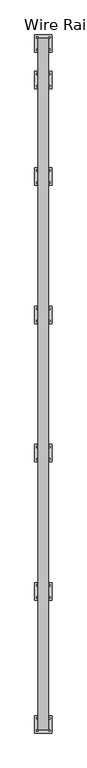
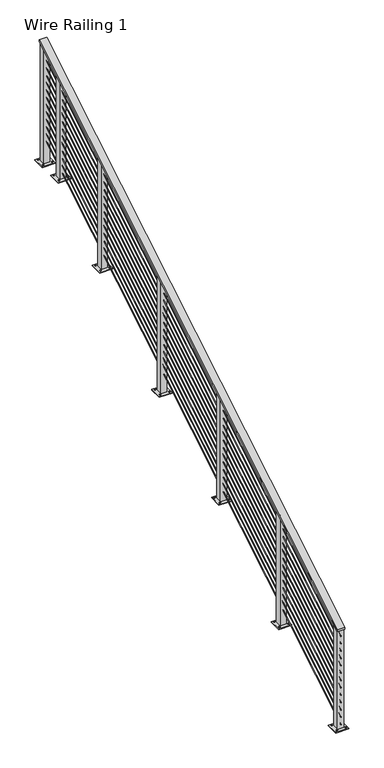
"""IFC4 building model written with IfcOpenShell, lengths in millimetres: railing geometry, Wire Railing 1."""

from ifc_helpers import new_model, si_unit, point, frame, frame_2d, origin, place, context, project, spatial, polyline, circle_curve, ellipse_curve, trimmed, segment, composite_curve, outline, extrude, faceted_brep, source, transform, mapped, element, save
from ifc_brep_helpers import plane_surface, cylinder_surface, advanced_brep


def wire_railing_1_93458223(model_context):
    return source(origin(), model_context, "Body", "SolidModel", [
        faceted_brep([(33186.6840778, 30205.3668167, 267463.590833), (33186.6840778, 30205.3668167, 267441.359167), (33262.8840778, 30205.3668167, 267441.359167), (33262.8840778, 30205.3668167, 267463.590833), (33186.6840778, 35259.9668167, 270504.4598169), (33262.8840778, 35259.9668167, 270504.4598169), (33262.8840778, 35259.9668167, 270482.228151), (33186.6840778, 35259.9668167, 270482.228151)], [[[0, 1, 2, 3]], [[4, 5, 6, 7]], [[1, 0, 4, 7]], [[2, 1, 7, 6]], [[3, 2, 6, 5]], [[0, 3, 5, 4]]]),
        advanced_brep(
        [(33227.1653278, 30205.3668167, 267383.0210418), (33222.4028278, 30205.3668167, 267383.0210418), (33227.1653278, 35259.9668167, 270423.8900257), (33222.4028278, 35259.9668167, 270423.8900257)],
        [
            (0, 1, ellipse_curve(frame((33224.7840778, 30205.3668167, 267383.0210418), z_axis=(0.0, -1.0, 0.0), x_axis=(0.0, 0.0, -1.0)), 2.7789582, 2.38125)),
            (1, 0, ellipse_curve(frame((33224.7840778, 30205.3668167, 267383.0210418), z_axis=(0.0, -1.0, 0.0), x_axis=(0.0, 0.0, -1.0)), 2.7789582, 2.38125)),
            (2, 3, ellipse_curve(frame((33224.7840778, 35259.9668167, 270423.8900257), z_axis=(0.0, 1.0, 0.0), x_axis=(0.0, 0.0, -1.0)), 2.7789582, 2.38125)),
            (3, 2, ellipse_curve(frame((33224.7840778, 35259.9668167, 270423.8900257), z_axis=(0.0, 1.0, 0.0), x_axis=(0.0, 0.0, -1.0)), 2.7789582, 2.38125)),
            (0, 2),
            (3, 1),
        ],
        [
            plane_surface(frame((33224.7840778, 30205.3668167, 267385.8), z_axis=(0.0, -1.0, 0.0), x_axis=(0.0, 0.0, 1.0))),
            plane_surface(frame((33224.7840778, 35259.9668167, 270426.668984), z_axis=(0.0, 1.0, 0.0), x_axis=(0.0, 0.0, 1.0))),
            cylinder_surface(frame((33224.7840778, 30206.5943658, 267383.7595406), z_axis=(0.0, -0.8568858520826472, -0.5155061944347475), x_axis=(-1.0, 0.0, 0.0)), 2.38125),
        ],
        [
            (0, [[1, 2]]),
            (1, [[3, 4]]),
            (2, [[-1, 5, -4, 6]]),
            (2, [[-2, -6, -3, -5]]),
        ],
    ),
        advanced_brep(
        [(33227.1653278, 30205.3668167, 267306.8210418), (33222.4028278, 30205.3668167, 267306.8210418), (33227.1653278, 35259.9668167, 270347.6900257), (33222.4028278, 35259.9668167, 270347.6900257)],
        [
            (0, 1, ellipse_curve(frame((33224.7840778, 30205.3668167, 267306.8210418), z_axis=(0.0, -1.0, 0.0), x_axis=(0.0, 0.0, -1.0)), 2.7789582, 2.38125)),
            (1, 0, ellipse_curve(frame((33224.7840778, 30205.3668167, 267306.8210418), z_axis=(0.0, -1.0, 0.0), x_axis=(0.0, 0.0, -1.0)), 2.7789582, 2.38125)),
            (2, 3, ellipse_curve(frame((33224.7840778, 35259.9668167, 270347.6900257), z_axis=(0.0, 1.0, 0.0), x_axis=(0.0, 0.0, -1.0)), 2.7789582, 2.38125)),
            (3, 2, ellipse_curve(frame((33224.7840778, 35259.9668167, 270347.6900257), z_axis=(0.0, 1.0, 0.0), x_axis=(0.0, 0.0, -1.0)), 2.7789582, 2.38125)),
            (0, 2),
            (3, 1),
        ],
        [
            plane_surface(frame((33224.7840778, 30205.3668167, 267309.6), z_axis=(0.0, -1.0, 0.0), x_axis=(0.0, 0.0, 1.0))),
            plane_surface(frame((33224.7840778, 35259.9668167, 270350.468984), z_axis=(0.0, 1.0, 0.0), x_axis=(0.0, 0.0, 1.0))),
            cylinder_surface(frame((33224.7840778, 30206.5943658, 267307.5595406), z_axis=(0.0, -0.8568858520826472, -0.5155061944347475), x_axis=(-1.0, 0.0, 0.0)), 2.38125),
        ],
        [
            (0, [[1, 2]]),
            (1, [[3, 4]]),
            (2, [[-1, 5, -4, 6]]),
            (2, [[-2, -6, -3, -5]]),
        ],
    ),
        advanced_brep(
        [(33227.1653278, 30205.3668167, 267230.6210418), (33222.4028278, 30205.3668167, 267230.6210418), (33227.1653278, 35259.9668167, 270271.4900257), (33222.4028278, 35259.9668167, 270271.4900257)],
        [
            (0, 1, ellipse_curve(frame((33224.7840778, 30205.3668167, 267230.6210418), z_axis=(0.0, -1.0, 0.0), x_axis=(0.0, 0.0, -1.0)), 2.7789582, 2.38125)),
            (1, 0, ellipse_curve(frame((33224.7840778, 30205.3668167, 267230.6210418), z_axis=(0.0, -1.0, 0.0), x_axis=(0.0, 0.0, -1.0)), 2.7789582, 2.38125)),
            (2, 3, ellipse_curve(frame((33224.7840778, 35259.9668167, 270271.4900257), z_axis=(0.0, 1.0, 0.0), x_axis=(0.0, 0.0, -1.0)), 2.7789582, 2.38125)),
            (3, 2, ellipse_curve(frame((33224.7840778, 35259.9668167, 270271.4900257), z_axis=(0.0, 1.0, 0.0), x_axis=(0.0, 0.0, -1.0)), 2.7789582, 2.38125)),
            (0, 2),
            (3, 1),
        ],
        [
            plane_surface(frame((33224.7840778, 30205.3668167, 267233.4), z_axis=(0.0, -1.0, 0.0), x_axis=(0.0, 0.0, 1.0))),
            plane_surface(frame((33224.7840778, 35259.9668167, 270274.268984), z_axis=(0.0, 1.0, 0.0), x_axis=(0.0, 0.0, 1.0))),
            cylinder_surface(frame((33224.7840778, 30206.5943658, 267231.3595406), z_axis=(0.0, -0.8568858520826472, -0.5155061944347475), x_axis=(-1.0, 0.0, 0.0)), 2.38125),
        ],
        [
            (0, [[1, 2]]),
            (1, [[3, 4]]),
            (2, [[-1, 5, -4, 6]]),
            (2, [[-2, -6, -3, -5]]),
        ],
    ),
        advanced_brep(
        [(33227.1653278, 30205.3668167, 267154.4210418), (33222.4028278, 30205.3668167, 267154.4210418), (33227.1653278, 35259.9668167, 270195.2900257), (33222.4028278, 35259.9668167, 270195.2900257)],
        [
            (0, 1, ellipse_curve(frame((33224.7840778, 30205.3668167, 267154.4210418), z_axis=(0.0, -1.0, 0.0), x_axis=(0.0, 0.0, -1.0)), 2.7789582, 2.38125)),
            (1, 0, ellipse_curve(frame((33224.7840778, 30205.3668167, 267154.4210418), z_axis=(0.0, -1.0, 0.0), x_axis=(0.0, 0.0, -1.0)), 2.7789582, 2.38125)),
            (2, 3, ellipse_curve(frame((33224.7840778, 35259.9668167, 270195.2900257), z_axis=(0.0, 1.0, 0.0), x_axis=(0.0, 0.0, -1.0)), 2.7789582, 2.38125)),
            (3, 2, ellipse_curve(frame((33224.7840778, 35259.9668167, 270195.2900257), z_axis=(0.0, 1.0, 0.0), x_axis=(0.0, 0.0, -1.0)), 2.7789582, 2.38125)),
            (0, 2),
            (3, 1),
        ],
        [
            plane_surface(frame((33224.7840778, 30205.3668167, 267157.2), z_axis=(0.0, -1.0, 0.0), x_axis=(0.0, 0.0, 1.0))),
            plane_surface(frame((33224.7840778, 35259.9668167, 270198.068984), z_axis=(0.0, 1.0, 0.0), x_axis=(0.0, 0.0, 1.0))),
            cylinder_surface(frame((33224.7840778, 30206.5943658, 267155.1595406), z_axis=(0.0, -0.8568858520826472, -0.5155061944347475), x_axis=(-1.0, 0.0, 0.0)), 2.38125),
        ],
        [
            (0, [[1, 2]]),
            (1, [[3, 4]]),
            (2, [[-1, 5, -4, 6]]),
            (2, [[-2, -6, -3, -5]]),
        ],
    ),
        advanced_brep(
        [(33227.1653278, 30205.3668167, 267078.2210418), (33222.4028278, 30205.3668167, 267078.2210418), (33227.1653278, 35259.9668167, 270119.0900257), (33222.4028278, 35259.9668167, 270119.0900257)],
        [
            (0, 1, ellipse_curve(frame((33224.7840778, 30205.3668167, 267078.2210418), z_axis=(0.0, -1.0, 0.0), x_axis=(0.0, 0.0, -1.0)), 2.7789582, 2.38125)),
            (1, 0, ellipse_curve(frame((33224.7840778, 30205.3668167, 267078.2210418), z_axis=(0.0, -1.0, 0.0), x_axis=(0.0, 0.0, -1.0)), 2.7789582, 2.38125)),
            (2, 3, ellipse_curve(frame((33224.7840778, 35259.9668167, 270119.0900257), z_axis=(0.0, 1.0, 0.0), x_axis=(0.0, 0.0, -1.0)), 2.7789582, 2.38125)),
            (3, 2, ellipse_curve(frame((33224.7840778, 35259.9668167, 270119.0900257), z_axis=(0.0, 1.0, 0.0), x_axis=(0.0, 0.0, -1.0)), 2.7789582, 2.38125)),
            (0, 2),
            (3, 1),
        ],
        [
            plane_surface(frame((33224.7840778, 30205.3668167, 267081.0), z_axis=(0.0, -1.0, 0.0), x_axis=(0.0, 0.0, 1.0))),
            plane_surface(frame((33224.7840778, 35259.9668167, 270121.868984), z_axis=(0.0, 1.0, 0.0), x_axis=(0.0, 0.0, 1.0))),
            cylinder_surface(frame((33224.7840778, 30206.5943658, 267078.9595406), z_axis=(0.0, -0.8568858520826472, -0.5155061944347475), x_axis=(-1.0, 0.0, 0.0)), 2.38125),
        ],
        [
            (0, [[1, 2]]),
            (1, [[3, 4]]),
            (2, [[-1, 5, -4, 6]]),
            (2, [[-2, -6, -3, -5]]),
        ],
    ),
        advanced_brep(
        [(33227.1653278, 30205.3668167, 267002.0210418), (33222.4028278, 30205.3668167, 267002.0210418), (33227.1653278, 35259.9668167, 270042.8900257), (33222.4028278, 35259.9668167, 270042.8900257)],
        [
            (0, 1, ellipse_curve(frame((33224.7840778, 30205.3668167, 267002.0210418), z_axis=(0.0, -1.0, 0.0), x_axis=(0.0, 0.0, -1.0)), 2.7789582, 2.38125)),
            (1, 0, ellipse_curve(frame((33224.7840778, 30205.3668167, 267002.0210418), z_axis=(0.0, -1.0, 0.0), x_axis=(0.0, 0.0, -1.0)), 2.7789582, 2.38125)),
            (2, 3, ellipse_curve(frame((33224.7840778, 35259.9668167, 270042.8900257), z_axis=(0.0, 1.0, 0.0), x_axis=(0.0, 0.0, -1.0)), 2.7789582, 2.38125)),
            (3, 2, ellipse_curve(frame((33224.7840778, 35259.9668167, 270042.8900257), z_axis=(0.0, 1.0, 0.0), x_axis=(0.0, 0.0, -1.0)), 2.7789582, 2.38125)),
            (0, 2),
            (3, 1),
        ],
        [
            plane_surface(frame((33224.7840778, 30205.3668167, 267004.8), z_axis=(0.0, -1.0, 0.0), x_axis=(0.0, 0.0, 1.0))),
            plane_surface(frame((33224.7840778, 35259.9668167, 270045.668984), z_axis=(0.0, 1.0, 0.0), x_axis=(0.0, 0.0, 1.0))),
            cylinder_surface(frame((33224.7840778, 30206.5943658, 267002.7595406), z_axis=(0.0, -0.8568858520826472, -0.5155061944347475), x_axis=(-1.0, 0.0, 0.0)), 2.38125),
        ],
        [
            (0, [[1, 2]]),
            (1, [[3, 4]]),
            (2, [[-1, 5, -4, 6]]),
            (2, [[-2, -6, -3, -5]]),
        ],
    ),
        advanced_brep(
        [(33227.1653278, 30205.3668167, 266925.8210418), (33222.4028278, 30205.3668167, 266925.8210418), (33227.1653278, 35259.9668167, 269966.6900257), (33222.4028278, 35259.9668167, 269966.6900257)],
        [
            (0, 1, ellipse_curve(frame((33224.7840778, 30205.3668167, 266925.8210418), z_axis=(0.0, -1.0, 0.0), x_axis=(0.0, 0.0, -1.0)), 2.7789582, 2.38125)),
            (1, 0, ellipse_curve(frame((33224.7840778, 30205.3668167, 266925.8210418), z_axis=(0.0, -1.0, 0.0), x_axis=(0.0, 0.0, -1.0)), 2.7789582, 2.38125)),
            (2, 3, ellipse_curve(frame((33224.7840778, 35259.9668167, 269966.6900257), z_axis=(0.0, 1.0, 0.0), x_axis=(0.0, 0.0, -1.0)), 2.7789582, 2.38125)),
            (3, 2, ellipse_curve(frame((33224.7840778, 35259.9668167, 269966.6900257), z_axis=(0.0, 1.0, 0.0), x_axis=(0.0, 0.0, -1.0)), 2.7789582, 2.38125)),
            (0, 2),
            (3, 1),
        ],
        [
            plane_surface(frame((33224.7840778, 30205.3668167, 266928.6), z_axis=(0.0, -1.0, 0.0), x_axis=(0.0, 0.0, 1.0))),
            plane_surface(frame((33224.7840778, 35259.9668167, 269969.468984), z_axis=(0.0, 1.0, 0.0), x_axis=(0.0, 0.0, 1.0))),
            cylinder_surface(frame((33224.7840778, 30206.5943658, 266926.5595406), z_axis=(0.0, -0.8568858520826472, -0.5155061944347475), x_axis=(-1.0, 0.0, 0.0)), 2.38125),
        ],
        [
            (0, [[1, 2]]),
            (1, [[3, 4]]),
            (2, [[-1, 5, -4, 6]]),
            (2, [[-2, -6, -3, -5]]),
        ],
    ),
        advanced_brep(
        [(33227.1653278, 30205.3668167, 266849.6210418), (33222.4028278, 30205.3668167, 266849.6210418), (33227.1653278, 35259.9668167, 269890.4900257), (33222.4028278, 35259.9668167, 269890.4900257)],
        [
            (0, 1, ellipse_curve(frame((33224.7840778, 30205.3668167, 266849.6210418), z_axis=(0.0, -1.0, 0.0), x_axis=(0.0, 0.0, -1.0)), 2.7789582, 2.38125)),
            (1, 0, ellipse_curve(frame((33224.7840778, 30205.3668167, 266849.6210418), z_axis=(0.0, -1.0, 0.0), x_axis=(0.0, 0.0, -1.0)), 2.7789582, 2.38125)),
            (2, 3, ellipse_curve(frame((33224.7840778, 35259.9668167, 269890.4900257), z_axis=(0.0, 1.0, 0.0), x_axis=(0.0, 0.0, -1.0)), 2.7789582, 2.38125)),
            (3, 2, ellipse_curve(frame((33224.7840778, 35259.9668167, 269890.4900257), z_axis=(0.0, 1.0, 0.0), x_axis=(0.0, 0.0, -1.0)), 2.7789582, 2.38125)),
            (0, 2),
            (3, 1),
        ],
        [
            plane_surface(frame((33224.7840778, 30205.3668167, 266852.4), z_axis=(0.0, -1.0, 0.0), x_axis=(0.0, 0.0, 1.0))),
            plane_surface(frame((33224.7840778, 35259.9668167, 269893.268984), z_axis=(0.0, 1.0, 0.0), x_axis=(0.0, 0.0, 1.0))),
            cylinder_surface(frame((33224.7840778, 30206.5943658, 266850.3595406), z_axis=(0.0, -0.8568858520826472, -0.5155061944347475), x_axis=(-1.0, 0.0, 0.0)), 2.38125),
        ],
        [
            (0, [[1, 2]]),
            (1, [[3, 4]]),
            (2, [[-1, 5, -4, 6]]),
            (2, [[-2, -6, -3, -5]]),
        ],
    ),
        advanced_brep(
        [(33227.1653278, 30205.3668167, 266773.4210418), (33222.4028278, 30205.3668167, 266773.4210418), (33227.1653278, 35259.9668167, 269814.2900257), (33222.4028278, 35259.9668167, 269814.2900257)],
        [
            (0, 1, ellipse_curve(frame((33224.7840778, 30205.3668167, 266773.4210418), z_axis=(0.0, -1.0, 0.0), x_axis=(0.0, 0.0, -1.0)), 2.7789582, 2.38125)),
            (1, 0, ellipse_curve(frame((33224.7840778, 30205.3668167, 266773.4210418), z_axis=(0.0, -1.0, 0.0), x_axis=(0.0, 0.0, -1.0)), 2.7789582, 2.38125)),
            (2, 3, ellipse_curve(frame((33224.7840778, 35259.9668167, 269814.2900257), z_axis=(0.0, 1.0, 0.0), x_axis=(0.0, 0.0, -1.0)), 2.7789582, 2.38125)),
            (3, 2, ellipse_curve(frame((33224.7840778, 35259.9668167, 269814.2900257), z_axis=(0.0, 1.0, 0.0), x_axis=(0.0, 0.0, -1.0)), 2.7789582, 2.38125)),
            (0, 2),
            (3, 1),
        ],
        [
            plane_surface(frame((33224.7840778, 30205.3668167, 266776.2), z_axis=(0.0, -1.0, 0.0), x_axis=(0.0, 0.0, 1.0))),
            plane_surface(frame((33224.7840778, 35259.9668167, 269817.068984), z_axis=(0.0, 1.0, 0.0), x_axis=(0.0, 0.0, 1.0))),
            cylinder_surface(frame((33224.7840778, 30206.5943658, 266774.1595406), z_axis=(0.0, -0.8568858520826472, -0.5155061944347475), x_axis=(-1.0, 0.0, 0.0)), 2.38125),
        ],
        [
            (0, [[1, 2]]),
            (1, [[3, 4]]),
            (2, [[-1, 5, -4, 6]]),
            (2, [[-2, -6, -3, -5]]),
        ],
    ),
        advanced_brep(
        [(33227.1653278, 30205.3668167, 266697.2210418), (33222.4028278, 30205.3668167, 266697.2210418), (33227.1653278, 35259.9668167, 269738.0900257), (33222.4028278, 35259.9668167, 269738.0900257)],
        [
            (0, 1, ellipse_curve(frame((33224.7840778, 30205.3668167, 266697.2210418), z_axis=(0.0, -1.0, 0.0), x_axis=(0.0, 0.0, -1.0)), 2.7789582, 2.38125)),
            (1, 0, ellipse_curve(frame((33224.7840778, 30205.3668167, 266697.2210418), z_axis=(0.0, -1.0, 0.0), x_axis=(0.0, 0.0, -1.0)), 2.7789582, 2.38125)),
            (2, 3, ellipse_curve(frame((33224.7840778, 35259.9668167, 269738.0900257), z_axis=(0.0, 1.0, 0.0), x_axis=(0.0, 0.0, -1.0)), 2.7789582, 2.38125)),
            (3, 2, ellipse_curve(frame((33224.7840778, 35259.9668167, 269738.0900257), z_axis=(0.0, 1.0, 0.0), x_axis=(0.0, 0.0, -1.0)), 2.7789582, 2.38125)),
            (0, 2),
            (3, 1),
        ],
        [
            plane_surface(frame((33224.7840778, 30205.3668167, 266700.0), z_axis=(0.0, -1.0, 0.0), x_axis=(0.0, 0.0, 1.0))),
            plane_surface(frame((33224.7840778, 35259.9668167, 269740.868984), z_axis=(0.0, 1.0, 0.0), x_axis=(0.0, 0.0, 1.0))),
            cylinder_surface(frame((33224.7840778, 30206.5943658, 266697.9595406), z_axis=(0.0, -0.8568858520826472, -0.5155061944347475), x_axis=(-1.0, 0.0, 0.0)), 2.38125),
        ],
        [
            (0, [[1, 2]]),
            (1, [[3, 4]]),
            (2, [[-1, 5, -4, 6]]),
            (2, [[-2, -6, -3, -5]]),
        ],
    ),
        advanced_brep(
        [(33227.1653278, 30205.3668167, 266621.0210418), (33222.4028278, 30205.3668167, 266621.0210418), (33227.1653278, 35259.9668167, 269661.8900257), (33222.4028278, 35259.9668167, 269661.8900257)],
        [
            (0, 1, ellipse_curve(frame((33224.7840778, 30205.3668167, 266621.0210418), z_axis=(0.0, -1.0, 0.0), x_axis=(0.0, 0.0, -1.0)), 2.7789582, 2.38125)),
            (1, 0, ellipse_curve(frame((33224.7840778, 30205.3668167, 266621.0210418), z_axis=(0.0, -1.0, 0.0), x_axis=(0.0, 0.0, -1.0)), 2.7789582, 2.38125)),
            (2, 3, ellipse_curve(frame((33224.7840778, 35259.9668167, 269661.8900257), z_axis=(0.0, 1.0, 0.0), x_axis=(0.0, 0.0, -1.0)), 2.7789582, 2.38125)),
            (3, 2, ellipse_curve(frame((33224.7840778, 35259.9668167, 269661.8900257), z_axis=(0.0, 1.0, 0.0), x_axis=(0.0, 0.0, -1.0)), 2.7789582, 2.38125)),
            (0, 2),
            (3, 1),
        ],
        [
            plane_surface(frame((33224.7840778, 30205.3668167, 266623.8), z_axis=(0.0, -1.0, 0.0), x_axis=(0.0, 0.0, 1.0))),
            plane_surface(frame((33224.7840778, 35259.9668167, 269664.668984), z_axis=(0.0, 1.0, 0.0), x_axis=(0.0, 0.0, 1.0))),
            cylinder_surface(frame((33224.7840778, 30206.5943658, 266621.7595406), z_axis=(0.0, -0.8568858520826472, -0.5155061944347475), x_axis=(-1.0, 0.0, 0.0)), 2.38125),
        ],
        [
            (0, [[1, 2]]),
            (1, [[3, 4]]),
            (2, [[-1, 5, -4, 6]]),
            (2, [[-2, -6, -3, -5]]),
        ],
    ),
        advanced_brep(
        [(33227.1653278, 30205.3668167, 266544.8210418), (33222.4028278, 30205.3668167, 266544.8210418), (33227.1653278, 35259.9668167, 269585.6900257), (33222.4028278, 35259.9668167, 269585.6900257)],
        [
            (0, 1, ellipse_curve(frame((33224.7840778, 30205.3668167, 266544.8210418), z_axis=(0.0, -1.0, 0.0), x_axis=(0.0, 0.0, -1.0)), 2.7789582, 2.38125)),
            (1, 0, ellipse_curve(frame((33224.7840778, 30205.3668167, 266544.8210418), z_axis=(0.0, -1.0, 0.0), x_axis=(0.0, 0.0, -1.0)), 2.7789582, 2.38125)),
            (2, 3, ellipse_curve(frame((33224.7840778, 35259.9668167, 269585.6900257), z_axis=(0.0, 1.0, 0.0), x_axis=(0.0, 0.0, -1.0)), 2.7789582, 2.38125)),
            (3, 2, ellipse_curve(frame((33224.7840778, 35259.9668167, 269585.6900257), z_axis=(0.0, 1.0, 0.0), x_axis=(0.0, 0.0, -1.0)), 2.7789582, 2.38125)),
            (0, 2),
            (3, 1),
        ],
        [
            plane_surface(frame((33224.7840778, 30205.3668167, 266547.6), z_axis=(0.0, -1.0, 0.0), x_axis=(0.0, 0.0, 1.0))),
            plane_surface(frame((33224.7840778, 35259.9668167, 269588.468984), z_axis=(0.0, 1.0, 0.0), x_axis=(0.0, 0.0, 1.0))),
            cylinder_surface(frame((33224.7840778, 30206.5943658, 266545.5595406), z_axis=(0.0, -0.8568858520826472, -0.5155061944347475), x_axis=(-1.0, 0.0, 0.0)), 2.38125),
        ],
        [
            (0, [[1, 2]]),
            (1, [[3, 4]]),
            (2, [[-1, 5, -4, 6]]),
            (2, [[-2, -6, -3, -5]]),
        ],
    ),
        advanced_brep(
        [(33227.1653278, 30205.3668167, 266468.6210418), (33222.4028278, 30205.3668167, 266468.6210418), (33227.1653278, 35259.9668167, 269509.4900257), (33222.4028278, 35259.9668167, 269509.4900257)],
        [
            (0, 1, ellipse_curve(frame((33224.7840778, 30205.3668167, 266468.6210418), z_axis=(0.0, -1.0, 0.0), x_axis=(0.0, 0.0, -1.0)), 2.7789582, 2.38125)),
            (1, 0, ellipse_curve(frame((33224.7840778, 30205.3668167, 266468.6210418), z_axis=(0.0, -1.0, 0.0), x_axis=(0.0, 0.0, -1.0)), 2.7789582, 2.38125)),
            (2, 3, ellipse_curve(frame((33224.7840778, 35259.9668167, 269509.4900257), z_axis=(0.0, 1.0, 0.0), x_axis=(0.0, 0.0, -1.0)), 2.7789582, 2.38125)),
            (3, 2, ellipse_curve(frame((33224.7840778, 35259.9668167, 269509.4900257), z_axis=(0.0, 1.0, 0.0), x_axis=(0.0, 0.0, -1.0)), 2.7789582, 2.38125)),
            (0, 2),
            (3, 1),
        ],
        [
            plane_surface(frame((33224.7840778, 30205.3668167, 266471.4), z_axis=(0.0, -1.0, 0.0), x_axis=(0.0, 0.0, 1.0))),
            plane_surface(frame((33224.7840778, 35259.9668167, 269512.268984), z_axis=(0.0, 1.0, 0.0), x_axis=(0.0, 0.0, 1.0))),
            cylinder_surface(frame((33224.7840778, 30206.5943658, 266469.3595406), z_axis=(0.0, -0.8568858520826472, -0.5155061944347475), x_axis=(-1.0, 0.0, 0.0)), 2.38125),
        ],
        [
            (0, [[1, 2]]),
            (1, [[3, 4]]),
            (2, [[-1, 5, -4, 6]]),
            (2, [[-2, -6, -3, -5]]),
        ],
    ),
        extrude(outline(composite_curve([segment(trimmed(circle_curve(frame_2d((33180.3340778, 34204.5968167)), 6.35), [point((33173.9840778, 34204.5968167))], [point((33186.6840778, 34204.5968167))], False, "CARTESIAN"), True, "CONTINUOUS"), segment(trimmed(circle_curve(frame_2d((33180.3340778, 34204.5968167)), 6.35), [point((33186.6840778, 34204.5968167))], [point((33173.9840778, 34204.5968167))], False, "CARTESIAN"), True, "CONTINUOUS")], self_intersect=False)), frame((0.0, 0.0, 268748.4352941), z_axis=(0.0, 0.0, 1.0), x_axis=(1.0, 0.0, 0.0)), (0.0, 0.0, 1.0), 12.7),
        extrude(outline(composite_curve([segment(trimmed(circle_curve(frame_2d((33269.2340778, 34204.5968167)), 6.35), [point((33262.8840778, 34204.5968167))], [point((33275.5840778, 34204.5968167))], False, "CARTESIAN"), True, "CONTINUOUS"), segment(trimmed(circle_curve(frame_2d((33269.2340778, 34204.5968167)), 6.35), [point((33275.5840778, 34204.5968167))], [point((33262.8840778, 34204.5968167))], False, "CARTESIAN"), True, "CONTINUOUS")], self_intersect=False)), frame((0.0, 0.0, 268748.4352941), z_axis=(0.0, 0.0, 1.0), x_axis=(1.0, 0.0, 0.0)), (0.0, 0.0, 1.0), 12.7),
        extrude(outline(composite_curve([segment(trimmed(circle_curve(frame_2d((33180.3340778, 34293.4968167)), 6.35), [point((33173.9840778, 34293.4968167))], [point((33186.6840778, 34293.4968167))], False, "CARTESIAN"), True, "CONTINUOUS"), segment(trimmed(circle_curve(frame_2d((33180.3340778, 34293.4968167)), 6.35), [point((33186.6840778, 34293.4968167))], [point((33173.9840778, 34293.4968167))], False, "CARTESIAN"), True, "CONTINUOUS")], self_intersect=False)), frame((0.0, 0.0, 268748.4352941), z_axis=(0.0, 0.0, 1.0), x_axis=(1.0, 0.0, 0.0)), (0.0, 0.0, 1.0), 12.7),
        extrude(outline(composite_curve([segment(trimmed(circle_curve(frame_2d((33269.2340778, 34293.4968167)), 6.35), [point((33262.8840778, 34293.4968167))], [point((33275.5840778, 34293.4968167))], False, "CARTESIAN"), True, "CONTINUOUS"), segment(trimmed(circle_curve(frame_2d((33269.2340778, 34293.4968167)), 6.35), [point((33275.5840778, 34293.4968167))], [point((33262.8840778, 34293.4968167))], False, "CARTESIAN"), True, "CONTINUOUS")], self_intersect=False)), frame((0.0, 0.0, 268748.4352941), z_axis=(0.0, 0.0, 1.0), x_axis=(1.0, 0.0, 0.0)), (0.0, 0.0, 1.0), 12.7),
        extrude(outline(polyline([(33288.2840778, 34185.5468167), (33161.2840778, 34185.5468167), (33161.2840778, 34312.5468167), (33288.2840778, 34312.5468167), (33288.2840778, 34185.5468167)])), frame((0.0, 0.0, 268748.4352941), z_axis=(0.0, 0.0, 1.0), x_axis=(1.0, 0.0, 0.0)), (0.0, 0.0, 1.0), 6.35),
        extrude(outline(polyline([(33254.9465778, 34218.8843167), (33194.6215778, 34218.8843167), (33194.6215778, 34279.2093167), (33254.9465778, 34279.2093167), (33254.9465778, 34218.8843167)]), holes=[polyline([(33248.5965778, 34225.2343167), (33248.5965778, 34272.8593167), (33200.9715778, 34272.8593167), (33200.9715778, 34225.2343167), (33248.5965778, 34225.2343167)])]), frame((0.0, 0.0, 268748.4352941), z_axis=(0.0, 0.0, 1.0), x_axis=(1.0, 0.0, 0.0)), (0.0, 0.0, 1.0), 1125.6190601),
        extrude(outline(composite_curve([segment(trimmed(circle_curve(frame_2d((33180.3340778, 33193.6768167)), 6.35), [point((33173.9840778, 33193.6768167))], [point((33186.6840778, 33193.6768167))], False, "CARTESIAN"), True, "CONTINUOUS"), segment(trimmed(circle_curve(frame_2d((33180.3340778, 33193.6768167)), 6.35), [point((33186.6840778, 33193.6768167))], [point((33173.9840778, 33193.6768167))], False, "CARTESIAN"), True, "CONTINUOUS")], self_intersect=False)), frame((0.0, 0.0, 268076.0823529), z_axis=(0.0, 0.0, 1.0), x_axis=(1.0, 0.0, 0.0)), (0.0, 0.0, 1.0), 12.7),
        extrude(outline(composite_curve([segment(trimmed(circle_curve(frame_2d((33269.2340778, 33193.6768167)), 6.35), [point((33262.8840778, 33193.6768167))], [point((33275.5840778, 33193.6768167))], False, "CARTESIAN"), True, "CONTINUOUS"), segment(trimmed(circle_curve(frame_2d((33269.2340778, 33193.6768167)), 6.35), [point((33275.5840778, 33193.6768167))], [point((33262.8840778, 33193.6768167))], False, "CARTESIAN"), True, "CONTINUOUS")], self_intersect=False)), frame((0.0, 0.0, 268076.0823529), z_axis=(0.0, 0.0, 1.0), x_axis=(1.0, 0.0, 0.0)), (0.0, 0.0, 1.0), 12.7),
        extrude(outline(composite_curve([segment(trimmed(circle_curve(frame_2d((33180.3340778, 33282.5768167)), 6.35), [point((33173.9840778, 33282.5768167))], [point((33186.6840778, 33282.5768167))], False, "CARTESIAN"), True, "CONTINUOUS"), segment(trimmed(circle_curve(frame_2d((33180.3340778, 33282.5768167)), 6.35), [point((33186.6840778, 33282.5768167))], [point((33173.9840778, 33282.5768167))], False, "CARTESIAN"), True, "CONTINUOUS")], self_intersect=False)), frame((0.0, 0.0, 268076.0823529), z_axis=(0.0, 0.0, 1.0), x_axis=(1.0, 0.0, 0.0)), (0.0, 0.0, 1.0), 12.7),
        extrude(outline(composite_curve([segment(trimmed(circle_curve(frame_2d((33269.2340778, 33282.5768167)), 6.35), [point((33262.8840778, 33282.5768167))], [point((33275.5840778, 33282.5768167))], False, "CARTESIAN"), True, "CONTINUOUS"), segment(trimmed(circle_curve(frame_2d((33269.2340778, 33282.5768167)), 6.35), [point((33275.5840778, 33282.5768167))], [point((33262.8840778, 33282.5768167))], False, "CARTESIAN"), True, "CONTINUOUS")], self_intersect=False)), frame((0.0, 0.0, 268076.0823529), z_axis=(0.0, 0.0, 1.0), x_axis=(1.0, 0.0, 0.0)), (0.0, 0.0, 1.0), 12.7),
        extrude(outline(polyline([(33288.2840778, 33174.6268167), (33161.2840778, 33174.6268167), (33161.2840778, 33301.6268167), (33288.2840778, 33301.6268167), (33288.2840778, 33174.6268167)])), frame((0.0, 0.0, 268076.0823529), z_axis=(0.0, 0.0, 1.0), x_axis=(1.0, 0.0, 0.0)), (0.0, 0.0, 1.0), 6.35),
        extrude(outline(polyline([(33254.9465778, 33207.9643167), (33194.6215778, 33207.9643167), (33194.6215778, 33268.2893167), (33254.9465778, 33268.2893167), (33254.9465778, 33207.9643167)]), holes=[polyline([(33248.5965778, 33214.3143167), (33248.5965778, 33261.9393167), (33200.9715778, 33261.9393167), (33200.9715778, 33214.3143167), (33248.5965778, 33214.3143167)])]), frame((0.0, 0.0, 268076.0823529), z_axis=(0.0, 0.0, 1.0), x_axis=(1.0, 0.0, 0.0)), (0.0, 0.0, 1.0), 1189.7982045),
        extrude(outline(composite_curve([segment(trimmed(circle_curve(frame_2d((33180.3340778, 32182.7568167)), 6.35), [point((33173.9840778, 32182.7568167))], [point((33186.6840778, 32182.7568167))], False, "CARTESIAN"), True, "CONTINUOUS"), segment(trimmed(circle_curve(frame_2d((33180.3340778, 32182.7568167)), 6.35), [point((33186.6840778, 32182.7568167))], [point((33173.9840778, 32182.7568167))], False, "CARTESIAN"), True, "CONTINUOUS")], self_intersect=False)), frame((0.0, 0.0, 267571.8176471), z_axis=(0.0, 0.0, 1.0), x_axis=(1.0, 0.0, 0.0)), (0.0, 0.0, 1.0), 12.7),
        extrude(outline(composite_curve([segment(trimmed(circle_curve(frame_2d((33269.2340778, 32182.7568167)), 6.35), [point((33262.8840778, 32182.7568167))], [point((33275.5840778, 32182.7568167))], False, "CARTESIAN"), True, "CONTINUOUS"), segment(trimmed(circle_curve(frame_2d((33269.2340778, 32182.7568167)), 6.35), [point((33275.5840778, 32182.7568167))], [point((33262.8840778, 32182.7568167))], False, "CARTESIAN"), True, "CONTINUOUS")], self_intersect=False)), frame((0.0, 0.0, 267571.8176471), z_axis=(0.0, 0.0, 1.0), x_axis=(1.0, 0.0, 0.0)), (0.0, 0.0, 1.0), 12.7),
        extrude(outline(composite_curve([segment(trimmed(circle_curve(frame_2d((33180.3340778, 32271.6568167)), 6.35), [point((33173.9840778, 32271.6568167))], [point((33186.6840778, 32271.6568167))], False, "CARTESIAN"), True, "CONTINUOUS"), segment(trimmed(circle_curve(frame_2d((33180.3340778, 32271.6568167)), 6.35), [point((33186.6840778, 32271.6568167))], [point((33173.9840778, 32271.6568167))], False, "CARTESIAN"), True, "CONTINUOUS")], self_intersect=False)), frame((0.0, 0.0, 267571.8176471), z_axis=(0.0, 0.0, 1.0), x_axis=(1.0, 0.0, 0.0)), (0.0, 0.0, 1.0), 12.7),
        extrude(outline(composite_curve([segment(trimmed(circle_curve(frame_2d((33269.2340778, 32271.6568167)), 6.35), [point((33262.8840778, 32271.6568167))], [point((33275.5840778, 32271.6568167))], False, "CARTESIAN"), True, "CONTINUOUS"), segment(trimmed(circle_curve(frame_2d((33269.2340778, 32271.6568167)), 6.35), [point((33275.5840778, 32271.6568167))], [point((33262.8840778, 32271.6568167))], False, "CARTESIAN"), True, "CONTINUOUS")], self_intersect=False)), frame((0.0, 0.0, 267571.8176471), z_axis=(0.0, 0.0, 1.0), x_axis=(1.0, 0.0, 0.0)), (0.0, 0.0, 1.0), 12.7),
        extrude(outline(polyline([(33288.2840778, 32163.7068167), (33161.2840778, 32163.7068167), (33161.2840778, 32290.7068167), (33288.2840778, 32290.7068167), (33288.2840778, 32163.7068167)])), frame((0.0, 0.0, 267571.8176471), z_axis=(0.0, 0.0, 1.0), x_axis=(1.0, 0.0, 0.0)), (0.0, 0.0, 1.0), 6.35),
        extrude(outline(polyline([(33254.9465778, 32197.0443167), (33194.6215778, 32197.0443167), (33194.6215778, 32257.3693167), (33254.9465778, 32257.3693167), (33254.9465778, 32197.0443167)]), holes=[polyline([(33248.5965778, 32203.3943167), (33248.5965778, 32251.0193167), (33200.9715778, 32251.0193167), (33200.9715778, 32203.3943167), (33248.5965778, 32203.3943167)])]), frame((0.0, 0.0, 267571.8176471), z_axis=(0.0, 0.0, 1.0), x_axis=(1.0, 0.0, 0.0)), (0.0, 0.0, 1.0), 1085.8891136),
        extrude(outline(composite_curve([segment(trimmed(circle_curve(frame_2d((33180.3340778, 31171.8368167)), 6.35), [point((33173.9840778, 31171.8368167))], [point((33186.6840778, 31171.8368167))], False, "CARTESIAN"), True, "CONTINUOUS"), segment(trimmed(circle_curve(frame_2d((33180.3340778, 31171.8368167)), 6.35), [point((33186.6840778, 31171.8368167))], [point((33173.9840778, 31171.8368167))], False, "CARTESIAN"), True, "CONTINUOUS")], self_intersect=False)), frame((0.0, 0.0, 266899.4647059), z_axis=(0.0, 0.0, 1.0), x_axis=(1.0, 0.0, 0.0)), (0.0, 0.0, 1.0), 12.7),
        extrude(outline(composite_curve([segment(trimmed(circle_curve(frame_2d((33269.2340778, 31171.8368167)), 6.35), [point((33262.8840778, 31171.8368167))], [point((33275.5840778, 31171.8368167))], False, "CARTESIAN"), True, "CONTINUOUS"), segment(trimmed(circle_curve(frame_2d((33269.2340778, 31171.8368167)), 6.35), [point((33275.5840778, 31171.8368167))], [point((33262.8840778, 31171.8368167))], False, "CARTESIAN"), True, "CONTINUOUS")], self_intersect=False)), frame((0.0, 0.0, 266899.4647059), z_axis=(0.0, 0.0, 1.0), x_axis=(1.0, 0.0, 0.0)), (0.0, 0.0, 1.0), 12.7),
        extrude(outline(composite_curve([segment(trimmed(circle_curve(frame_2d((33180.3340778, 31260.7368167)), 6.35), [point((33173.9840778, 31260.7368167))], [point((33186.6840778, 31260.7368167))], False, "CARTESIAN"), True, "CONTINUOUS"), segment(trimmed(circle_curve(frame_2d((33180.3340778, 31260.7368167)), 6.35), [point((33186.6840778, 31260.7368167))], [point((33173.9840778, 31260.7368167))], False, "CARTESIAN"), True, "CONTINUOUS")], self_intersect=False)), frame((0.0, 0.0, 266899.4647059), z_axis=(0.0, 0.0, 1.0), x_axis=(1.0, 0.0, 0.0)), (0.0, 0.0, 1.0), 12.7),
        extrude(outline(composite_curve([segment(trimmed(circle_curve(frame_2d((33269.2340778, 31260.7368167)), 6.35), [point((33262.8840778, 31260.7368167))], [point((33275.5840778, 31260.7368167))], False, "CARTESIAN"), True, "CONTINUOUS"), segment(trimmed(circle_curve(frame_2d((33269.2340778, 31260.7368167)), 6.35), [point((33275.5840778, 31260.7368167))], [point((33262.8840778, 31260.7368167))], False, "CARTESIAN"), True, "CONTINUOUS")], self_intersect=False)), frame((0.0, 0.0, 266899.4647059), z_axis=(0.0, 0.0, 1.0), x_axis=(1.0, 0.0, 0.0)), (0.0, 0.0, 1.0), 12.7),
        extrude(outline(polyline([(33288.2840778, 31152.7868167), (33161.2840778, 31152.7868167), (33161.2840778, 31279.7868167), (33288.2840778, 31279.7868167), (33288.2840778, 31152.7868167)])), frame((0.0, 0.0, 266899.4647059), z_axis=(0.0, 0.0, 1.0), x_axis=(1.0, 0.0, 0.0)), (0.0, 0.0, 1.0), 6.35),
        extrude(outline(polyline([(33254.9465778, 31186.1243167), (33194.6215778, 31186.1243167), (33194.6215778, 31246.4493167), (33254.9465778, 31246.4493167), (33254.9465778, 31186.1243167)]), holes=[polyline([(33248.5965778, 31192.4743167), (33248.5965778, 31240.0993167), (33200.9715778, 31240.0993167), (33200.9715778, 31192.4743167), (33248.5965778, 31192.4743167)])]), frame((0.0, 0.0, 266899.4647059), z_axis=(0.0, 0.0, 1.0), x_axis=(1.0, 0.0, 0.0)), (0.0, 0.0, 1.0), 1150.0682579),
        extrude(outline(composite_curve([segment(trimmed(circle_curve(frame_2d((33180.3340778, 34910.7168167)), 6.35), [point((33173.9840778, 34910.7168167))], [point((33186.6840778, 34910.7168167))], False, "CARTESIAN"), True, "CONTINUOUS"), segment(trimmed(circle_curve(frame_2d((33180.3340778, 34910.7168167)), 6.35), [point((33186.6840778, 34910.7168167))], [point((33173.9840778, 34910.7168167))], False, "CARTESIAN"), True, "CONTINUOUS")], self_intersect=False)), frame((0.0, 0.0, 269252.7), z_axis=(0.0, 0.0, 1.0), x_axis=(1.0, 0.0, 0.0)), (0.0, 0.0, 1.0), 12.7),
        extrude(outline(composite_curve([segment(trimmed(circle_curve(frame_2d((33269.2340778, 34910.7168167)), 6.35), [point((33262.8840778, 34910.7168167))], [point((33275.5840778, 34910.7168167))], False, "CARTESIAN"), True, "CONTINUOUS"), segment(trimmed(circle_curve(frame_2d((33269.2340778, 34910.7168167)), 6.35), [point((33275.5840778, 34910.7168167))], [point((33262.8840778, 34910.7168167))], False, "CARTESIAN"), True, "CONTINUOUS")], self_intersect=False)), frame((0.0, 0.0, 269252.7), z_axis=(0.0, 0.0, 1.0), x_axis=(1.0, 0.0, 0.0)), (0.0, 0.0, 1.0), 12.7),
        extrude(outline(composite_curve([segment(trimmed(circle_curve(frame_2d((33180.3340778, 34999.6168167)), 6.35), [point((33173.9840778, 34999.6168167))], [point((33186.6840778, 34999.6168167))], False, "CARTESIAN"), True, "CONTINUOUS"), segment(trimmed(circle_curve(frame_2d((33180.3340778, 34999.6168167)), 6.35), [point((33186.6840778, 34999.6168167))], [point((33173.9840778, 34999.6168167))], False, "CARTESIAN"), True, "CONTINUOUS")], self_intersect=False)), frame((0.0, 0.0, 269252.7), z_axis=(0.0, 0.0, 1.0), x_axis=(1.0, 0.0, 0.0)), (0.0, 0.0, 1.0), 12.7),
        extrude(outline(composite_curve([segment(trimmed(circle_curve(frame_2d((33269.2340778, 34999.6168167)), 6.35), [point((33262.8840778, 34999.6168167))], [point((33275.5840778, 34999.6168167))], False, "CARTESIAN"), True, "CONTINUOUS"), segment(trimmed(circle_curve(frame_2d((33269.2340778, 34999.6168167)), 6.35), [point((33275.5840778, 34999.6168167))], [point((33262.8840778, 34999.6168167))], False, "CARTESIAN"), True, "CONTINUOUS")], self_intersect=False)), frame((0.0, 0.0, 269252.7), z_axis=(0.0, 0.0, 1.0), x_axis=(1.0, 0.0, 0.0)), (0.0, 0.0, 1.0), 12.7),
        extrude(outline(polyline([(33288.2840778, 34891.6668167), (33161.2840778, 34891.6668167), (33161.2840778, 35018.6668167), (33288.2840778, 35018.6668167), (33288.2840778, 34891.6668167)])), frame((0.0, 0.0, 269252.7), z_axis=(0.0, 0.0, 1.0), x_axis=(1.0, 0.0, 0.0)), (0.0, 0.0, 1.0), 6.35),
        extrude(outline(polyline([(33254.9465778, 34925.0043167), (33194.6215778, 34925.0043167), (33194.6215778, 34985.3293167), (33254.9465778, 34985.3293167), (33254.9465778, 34925.0043167)]), holes=[polyline([(33248.5965778, 34931.3543167), (33248.5965778, 34978.9793167), (33200.9715778, 34978.9793167), (33200.9715778, 34931.3543167), (33248.5965778, 34931.3543167)])]), frame((0.0, 0.0, 269252.7), z_axis=(0.0, 0.0, 1.0), x_axis=(1.0, 0.0, 0.0)), (0.0, 0.0, 1.0), 1046.159167),
        extrude(outline(composite_curve([segment(trimmed(circle_curve(frame_2d((33180.3340778, 35177.4168167)), 6.35), [point((33173.9840778, 35177.4168167))], [point((33186.6840778, 35177.4168167))], False, "CARTESIAN"), True, "CONTINUOUS"), segment(trimmed(circle_curve(frame_2d((33180.3340778, 35177.4168167)), 6.35), [point((33186.6840778, 35177.4168167))], [point((33173.9840778, 35177.4168167))], False, "CARTESIAN"), True, "CONTINUOUS")], self_intersect=False)), frame((0.0, 0.0, 269252.7), z_axis=(0.0, 0.0, 1.0), x_axis=(1.0, 0.0, 0.0)), (0.0, 0.0, 1.0), 12.7),
        extrude(outline(composite_curve([segment(trimmed(circle_curve(frame_2d((33269.2340778, 35177.4168167)), 6.35), [point((33262.8840778, 35177.4168167))], [point((33275.5840778, 35177.4168167))], False, "CARTESIAN"), True, "CONTINUOUS"), segment(trimmed(circle_curve(frame_2d((33269.2340778, 35177.4168167)), 6.35), [point((33275.5840778, 35177.4168167))], [point((33262.8840778, 35177.4168167))], False, "CARTESIAN"), True, "CONTINUOUS")], self_intersect=False)), frame((0.0, 0.0, 269252.7), z_axis=(0.0, 0.0, 1.0), x_axis=(1.0, 0.0, 0.0)), (0.0, 0.0, 1.0), 12.7),
        extrude(outline(composite_curve([segment(trimmed(circle_curve(frame_2d((33180.3340778, 35266.3168167)), 6.35), [point((33173.9840778, 35266.3168167))], [point((33186.6840778, 35266.3168167))], False, "CARTESIAN"), True, "CONTINUOUS"), segment(trimmed(circle_curve(frame_2d((33180.3340778, 35266.3168167)), 6.35), [point((33186.6840778, 35266.3168167))], [point((33173.9840778, 35266.3168167))], False, "CARTESIAN"), True, "CONTINUOUS")], self_intersect=False)), frame((0.0, 0.0, 269252.7), z_axis=(0.0, 0.0, 1.0), x_axis=(1.0, 0.0, 0.0)), (0.0, 0.0, 1.0), 12.7),
        extrude(outline(composite_curve([segment(trimmed(circle_curve(frame_2d((33269.2340778, 35266.3168167)), 6.35), [point((33262.8840778, 35266.3168167))], [point((33275.5840778, 35266.3168167))], False, "CARTESIAN"), True, "CONTINUOUS"), segment(trimmed(circle_curve(frame_2d((33269.2340778, 35266.3168167)), 6.35), [point((33275.5840778, 35266.3168167))], [point((33262.8840778, 35266.3168167))], False, "CARTESIAN"), True, "CONTINUOUS")], self_intersect=False)), frame((0.0, 0.0, 269252.7), z_axis=(0.0, 0.0, 1.0), x_axis=(1.0, 0.0, 0.0)), (0.0, 0.0, 1.0), 12.7),
        extrude(outline(polyline([(33288.2840778, 35158.3668167), (33161.2840778, 35158.3668167), (33161.2840778, 35285.3668167), (33288.2840778, 35285.3668167), (33288.2840778, 35158.3668167)])), frame((0.0, 0.0, 269252.7), z_axis=(0.0, 0.0, 1.0), x_axis=(1.0, 0.0, 0.0)), (0.0, 0.0, 1.0), 6.35),
        extrude(outline(polyline([(33254.9465778, 35191.7043167), (33194.6215778, 35191.7043167), (33194.6215778, 35252.0293167), (33254.9465778, 35252.0293167), (33254.9465778, 35191.7043167)]), holes=[polyline([(33248.5965778, 35198.0543167), (33248.5965778, 35245.6793167), (33200.9715778, 35245.6793167), (33200.9715778, 35198.0543167), (33248.5965778, 35198.0543167)])]), frame((0.0, 0.0, 269252.7), z_axis=(0.0, 0.0, 1.0), x_axis=(1.0, 0.0, 0.0)), (0.0, 0.0, 1.0), 1206.607028),
        extrude(outline(composite_curve([segment(trimmed(circle_curve(frame_2d((33180.3340778, 30199.0168167)), 6.35), [point((33173.9840778, 30199.0168167))], [point((33186.6840778, 30199.0168167))], False, "CARTESIAN"), True, "CONTINUOUS"), segment(trimmed(circle_curve(frame_2d((33180.3340778, 30199.0168167)), 6.35), [point((33186.6840778, 30199.0168167))], [point((33173.9840778, 30199.0168167))], False, "CARTESIAN"), True, "CONTINUOUS")], self_intersect=False)), frame((0.0, 0.0, 266418.121123), z_axis=(0.0, 0.0, 1.0), x_axis=(1.0, 0.0, 0.0)), (0.0, 0.0, 1.0), 12.7),
        extrude(outline(composite_curve([segment(trimmed(circle_curve(frame_2d((33269.2340778, 30199.0168167)), 6.35), [point((33262.8840778, 30199.0168167))], [point((33275.5840778, 30199.0168167))], False, "CARTESIAN"), True, "CONTINUOUS"), segment(trimmed(circle_curve(frame_2d((33269.2340778, 30199.0168167)), 6.35), [point((33275.5840778, 30199.0168167))], [point((33262.8840778, 30199.0168167))], False, "CARTESIAN"), True, "CONTINUOUS")], self_intersect=False)), frame((0.0, 0.0, 266418.121123), z_axis=(0.0, 0.0, 1.0), x_axis=(1.0, 0.0, 0.0)), (0.0, 0.0, 1.0), 12.7),
        extrude(outline(composite_curve([segment(trimmed(circle_curve(frame_2d((33180.3340778, 30287.9168167)), 6.35), [point((33173.9840778, 30287.9168167))], [point((33186.6840778, 30287.9168167))], False, "CARTESIAN"), True, "CONTINUOUS"), segment(trimmed(circle_curve(frame_2d((33180.3340778, 30287.9168167)), 6.35), [point((33186.6840778, 30287.9168167))], [point((33173.9840778, 30287.9168167))], False, "CARTESIAN"), True, "CONTINUOUS")], self_intersect=False)), frame((0.0, 0.0, 266418.121123), z_axis=(0.0, 0.0, 1.0), x_axis=(1.0, 0.0, 0.0)), (0.0, 0.0, 1.0), 12.7),
        extrude(outline(composite_curve([segment(trimmed(circle_curve(frame_2d((33269.2340778, 30287.9168167)), 6.35), [point((33262.8840778, 30287.9168167))], [point((33275.5840778, 30287.9168167))], False, "CARTESIAN"), True, "CONTINUOUS"), segment(trimmed(circle_curve(frame_2d((33269.2340778, 30287.9168167)), 6.35), [point((33275.5840778, 30287.9168167))], [point((33262.8840778, 30287.9168167))], False, "CARTESIAN"), True, "CONTINUOUS")], self_intersect=False)), frame((0.0, 0.0, 266418.121123), z_axis=(0.0, 0.0, 1.0), x_axis=(1.0, 0.0, 0.0)), (0.0, 0.0, 1.0), 12.7),
        extrude(outline(polyline([(33288.2840778, 30179.9668167), (33161.2840778, 30179.9668167), (33161.2840778, 30306.9668167), (33288.2840778, 30306.9668167), (33288.2840778, 30179.9668167)])), frame((0.0, 0.0, 266418.121123), z_axis=(0.0, 0.0, 1.0), x_axis=(1.0, 0.0, 0.0)), (0.0, 0.0, 1.0), 6.35),
        extrude(outline(polyline([(33254.9465778, 30213.3043167), (33194.6215778, 30213.3043167), (33194.6215778, 30273.6293167), (33254.9465778, 30273.6293167), (33254.9465778, 30213.3043167)]), holes=[polyline([(33248.5965778, 30219.6543167), (33248.5965778, 30267.2793167), (33200.9715778, 30267.2793167), (33200.9715778, 30219.6543167), (33248.5965778, 30219.6543167)])]), frame((0.0, 0.0, 266418.121123), z_axis=(0.0, 0.0, 1.0), x_axis=(1.0, 0.0, 0.0)), (0.0, 0.0, 1.0), 1046.159167),
    ])


if __name__ == "__main__":
    model = new_model("IFC4")
    model_context = context("Model", 3, world=origin())
    ifc_project = project(units=[si_unit("LENGTHUNIT", "METRE", prefix="MILLI")], contexts=[model_context])
    site = spatial("IfcSite", under=ifc_project)
    building = spatial("IfcBuilding", under=site)
    placement = place(None, origin())
    wire_railing_1_shape = wire_railing_1_93458223(model_context)
    element("IfcRailing", 1, ObjectType="Wire Railing 1", at=placement, inside=building, context=model_context, shape_type="MappedRepresentation", body=[
        mapped(wire_railing_1_shape, transform((0.0, 0.0, 0.0), x_axis=(1.0, 0.0, 0.0), y_axis=(0.0, 1.0, 0.0), z_axis=(0.0, 0.0, 1.0))),
    ])
    save(model, "model.ifc")

# Revit data of these elements
# Element 1 (IfcRailing, "Wire Railing 1")
#   Materials on its faces: "WIRE RAILING"
# Materials
#   "WIRE RAILING": class "Metal", colour RGB 244 244 244, transparency 0, Manufacturer = "Kawneer", URL = "http://www.kawneer.com/kawneer/north_america/en/home.asp", Cost = 0
